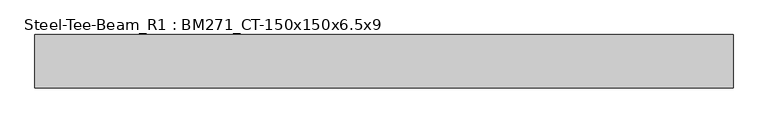
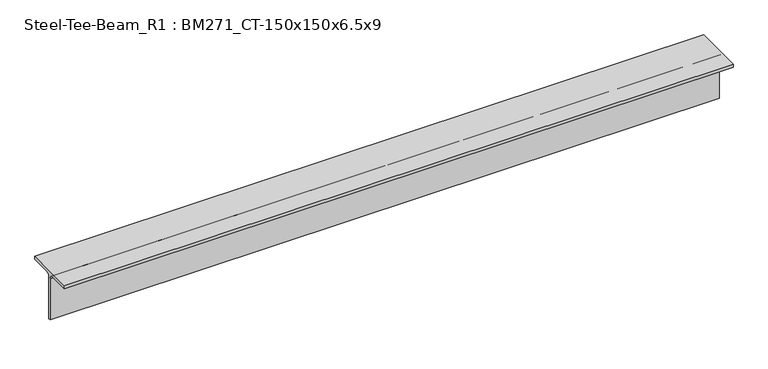
"""IFC4 building model written with IfcOpenShell, lengths in millimetres: member geometry, Steel-Tee-Beam_R1 : BM271_CT-150x150x6.5x9."""

from ifc_helpers import new_model, si_unit, point, frame, frame_2d, origin, place, context, project, spatial, polyline, circle_curve, trimmed, segment, composite_curve, outline, extrude, source, transform, mapped, element, save


def steel_tee_beam_r1_bm271_ct_150x150x6_5x9_f0f58029(model_context):
    return source(origin(), model_context, "Body", "SweptSolid", [
        extrude(outline(composite_curve([segment(polyline([(-75.0, 75.0), (75.0, 75.0), (75.0, 66.0), (16.25, 66.0)]), True, "CONTINUOUS"), segment(trimmed(circle_curve(frame_2d((16.25, 53.0)), 13.0), [point((16.25, 66.0))], [point((3.25, 53.0))], True, "CARTESIAN"), True, "CONTINUOUS"), segment(polyline([(3.25, 53.0), (3.25, -75.0), (-3.25, -75.0), (-3.25, 53.0)]), True, "CONTINUOUS"), segment(trimmed(circle_curve(frame_2d((-16.25, 53.0)), 13.0), [point((-3.25, 53.0))], [point((-16.25, 66.0))], True, "CARTESIAN"), True, "CONTINUOUS"), segment(polyline([(-16.25, 66.0), (-75.0, 66.0), (-75.0, 75.0)]), True, "CONTINUOUS")], self_intersect=False)), frame((-1124.1990532, 0.0, 0.0), z_axis=(1.0, 0.0, 0.0), x_axis=(0.0, 1.0, 0.0)), (0.0, 0.0, 1.0), 1966.5219512),
    ])


if __name__ == "__main__":
    model = new_model("IFC4")
    model_context = context("Model", 3, world=origin())
    ifc_project = project(units=[si_unit("LENGTHUNIT", "METRE", prefix="MILLI")], contexts=[model_context])
    site = spatial("IfcSite", under=ifc_project)
    building = spatial("IfcBuilding", under=site)
    placement = place(None, origin())
    steel_tee_beam_r1_bm271_ct_150x150x6_5x9_shape = steel_tee_beam_r1_bm271_ct_150x150x6_5x9_f0f58029(model_context)
    element("IfcMember", 1, ObjectType="Steel-Tee-Beam_R1 : BM271_CT-150x150x6.5x9", at=placement, inside=building, context=model_context, shape_type="MappedRepresentation", body=[
        mapped(steel_tee_beam_r1_bm271_ct_150x150x6_5x9_shape, transform((0.0, 0.0, 0.0), x_axis=(1.0, 0.0, 0.0), y_axis=(0.0, 1.0, 0.0), z_axis=(0.0, 0.0, 1.0))),
    ])
    save(model, "model.ifc")

# Revit data of these elements
# Type "Steel-Tee-Beam_R1 : BM271_CT-150x150x6.5x9"
#   Keynote = "CT-150x150x6.5x9"
#   Surface Area = 0.588841 m²/m
#   Section Area = 23.3904 cm²
#   Mass per Unit Length = 18.3614 kg/m
#   Length [instance default] = 1.5240 m
#   bf = 0.1500 m
#   d = 0.1500 m
#   k = 0.0220 m
#   r = 0.0130 m
#   tf = 0.0090 m
#   tw = 0.0065 m
#   hec_material4 [instance default] = none
#   hec_material3 [instance default] = none
#   hec_material2 [instance default] = none
#   hec_material1 [instance default] = none
#   Structural Material [instance default] = Steel, 45-345
#   Assembly Code = ""
# Element 1 (IfcMember, "Steel-Tee-Beam_R1 : BM271_CT-150x150x6.5x9")
#   Structural Material = none
# Materials
#   "Steel, 45-345": class "Metal", colour RGB 189 187 185, transparency 0, Description = "Steel 345 MPa", Cost = 0
